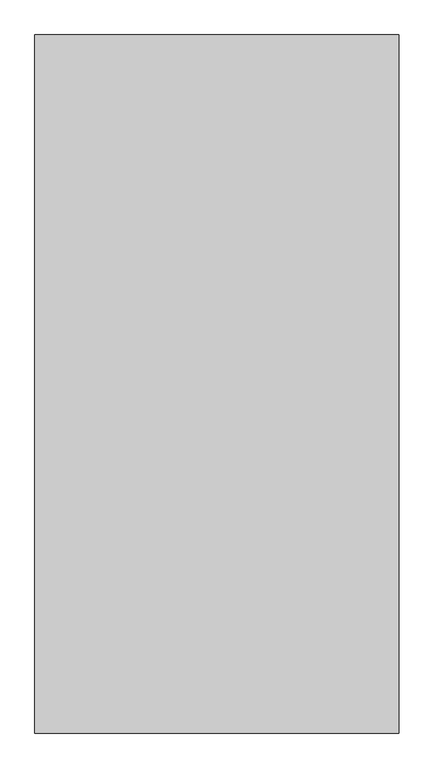
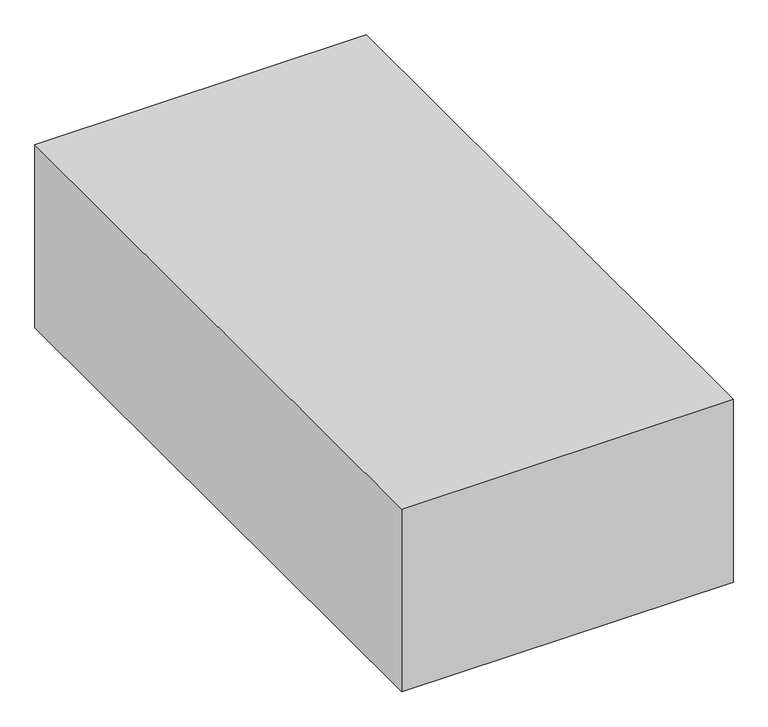
"""IFC4 building model written with IfcOpenShell, lengths in millimetres: proxy geometry, Space Planning Box_hec : Space Planning Box_hec."""

import ifcopenshell
import ifcopenshell.guid

model = None  # the IFC model being written
_history = None  # IfcOwnerHistory: only IFC2X3 demands one
_inside = {}  # id of a spatial element -> (the spatial element, [elements in it])
_under = {}  # id of a project, library or spatial element -> (it, [spatial elements below it])
_declared = {}  # id of a project -> (the project, [libraries it declares])
_typed = {}  # id of a type object -> (the type object, [elements of that type])
_made_of = {}  # id of a material, layer set ... -> (it, [elements and type objects made of it])


def new_model(schema):
    """Start an empty IFC model of exactly this schema.

    Asked for "IFC4X3", IfcOpenShell would pick the latest addendum, in which some entities
    have other attributes; the version numbers below select the first issue.
    IFC2X3 requires an IfcOwnerHistory on every rooted entity: one is made here for all.
    """
    global model, _history
    if schema == "IFC4X3":
        model = ifcopenshell.file(schema_version=(4, 3, 0, 0))
    else:
        model = ifcopenshell.file(schema=schema)
    _inside.clear()
    _under.clear()
    _declared.clear()
    _typed.clear()
    _made_of.clear()
    _history = None
    if model.schema == "IFC2X3":
        org = make("IfcOrganization", Name="unknown")
        user = make(
            "IfcPersonAndOrganization",
            ThePerson=make("IfcPerson", FamilyName="unknown"),
            TheOrganization=org,
        )
        app = make(
            "IfcApplication",
            ApplicationDeveloper=org,
            Version="unknown",
            ApplicationFullName="unknown",
            ApplicationIdentifier="unknown",
        )
        _history = make(
            "IfcOwnerHistory",
            OwningUser=user,
            OwningApplication=app,
            ChangeAction="ADDED",
            CreationDate=0,
        )
    return model


def make(cls, **values):
    """One entity of the class cls with the attributes given. An attribute that is None is left unset."""
    return model.create_entity(
        cls, **{name: value for name, value in values.items() if value is not None}
    )


def rooted(cls, **values):
    """An entity with a GlobalId (a new one), such as an element, a storey or a relation."""
    return make(cls, GlobalId=ifcopenshell.guid.new(), OwnerHistory=_history, **values)


def si_unit(unit_type, name, prefix=None):
    """IfcSIUnit, for example si_unit("LENGTHUNIT", "METRE", prefix="MILLI")."""
    return make("IfcSIUnit", UnitType=unit_type, Prefix=prefix, Name=name)


def assignment(units):
    """IfcUnitAssignment: the units of a project."""
    return None if units is None else make("IfcUnitAssignment", Units=units)


def point(xyz):
    """IfcCartesianPoint."""
    return None if xyz is None else make("IfcCartesianPoint", Coordinates=xyz)


def direction(xyz):
    """IfcDirection."""
    return None if xyz is None else make("IfcDirection", DirectionRatios=xyz)


def frame(location, z_axis=None, x_axis=None):
    """IfcAxis2Placement3D, a coordinate frame: its origin and axes. An axis left out is left unset."""
    return make(
        "IfcAxis2Placement3D",
        Location=point(location),
        Axis=direction(z_axis),
        RefDirection=direction(x_axis),
    )


def origin():
    """The frame at (0, 0, 0) with its axes left unset."""
    return frame((0.0, 0.0, 0.0))


def origin_with_axes():
    """The frame at (0, 0, 0) with the z axis (0, 0, 1) and the x axis (1, 0, 0) written out."""
    return frame((0.0, 0.0, 0.0), z_axis=(0.0, 0.0, 1.0), x_axis=(1.0, 0.0, 0.0))


def place(relative_to, where):
    """IfcLocalPlacement: puts the frame where relative to a parent placement (None: the world)."""
    return make(
        "IfcLocalPlacement", PlacementRelTo=relative_to, RelativePlacement=where
    )


def context(
    kind, dimensions, precision=None, world=None, true_north=None, identifier=None
):
    """IfcGeometricRepresentationContext, for example the 3D "Model" context."""
    return make(
        "IfcGeometricRepresentationContext",
        ContextIdentifier=identifier,
        ContextType=kind,
        CoordinateSpaceDimension=dimensions,
        Precision=precision,
        WorldCoordinateSystem=world,
        TrueNorth=true_north,
    )


def project(units=None, contexts=None):
    """IfcProject with its units and contexts."""
    return rooted(
        "IfcProject",
        Name="project",
        RepresentationContexts=contexts,
        UnitsInContext=assignment(units),
    )


def spatial(cls, under=None, at=None, **own):
    """A site, building, storey or space (cls), placed at a placement, below another one or the project."""
    s = rooted(cls, ObjectPlacement=at, **own)
    if under is not None:
        _under.setdefault(under.id(), (under, []))[1].append(s)
    return s


def polyline(points):
    """IfcPolyline through the points."""
    return make("IfcPolyline", Points=[point(p) for p in points])


def outline(outer, holes=None, kind="AREA"):
    """IfcArbitraryClosedProfileDef: a profile drawn as a closed curve; with holes, ...WithVoids."""
    if holes is None:
        return make("IfcArbitraryClosedProfileDef", ProfileType=kind, OuterCurve=outer)
    return make(
        "IfcArbitraryProfileDefWithVoids",
        ProfileType=kind,
        OuterCurve=outer,
        InnerCurves=holes,
    )


def extrude(swept, where, along, depth):
    """IfcExtrudedAreaSolid: the profile swept, set in the frame where, extruded along a direction by depth."""
    return make(
        "IfcExtrudedAreaSolid",
        SweptArea=swept,
        Position=where,
        ExtrudedDirection=direction(along),
        Depth=depth,
    )


def shape(context_of_items, identifier, shape_type, items):
    """IfcShapeRepresentation: the items that make up one representation, for example the "Body"."""
    return make(
        "IfcShapeRepresentation",
        ContextOfItems=context_of_items,
        RepresentationIdentifier=identifier,
        RepresentationType=shape_type,
        Items=items,
    )


def source(mapping_origin, context_of_items, identifier, shape_type, items):
    """IfcRepresentationMap: a shape defined once, which mapped items show again and again."""
    return make(
        "IfcRepresentationMap",
        MappingOrigin=mapping_origin,
        MappedRepresentation=shape(context_of_items, identifier, shape_type, items),
    )


def transform(
    local_origin,
    x_axis=None,
    y_axis=None,
    z_axis=None,
    scale=None,
    scale2=None,
    scale3=None,
    uniform=True,
):
    """IfcCartesianTransformationOperator3D, or its non-uniform kind. x_axis, y_axis, z_axis: its Axis1, 2, 3."""
    if uniform:
        return make(
            "IfcCartesianTransformationOperator3D",
            Axis1=direction(x_axis),
            Axis2=direction(y_axis),
            LocalOrigin=point(local_origin),
            Scale=scale,
            Axis3=direction(z_axis),
        )
    return make(
        "IfcCartesianTransformationOperator3DnonUniform",
        Axis1=direction(x_axis),
        Axis2=direction(y_axis),
        LocalOrigin=point(local_origin),
        Scale=scale,
        Axis3=direction(z_axis),
        Scale2=scale2,
        Scale3=scale3,
    )


def mapped(mapping_source, mapping_target):
    """IfcMappedItem: shows the shape of a source again, moved by a transform."""
    return make(
        "IfcMappedItem", MappingSource=mapping_source, MappingTarget=mapping_target
    )


def made_of(thing, what):
    """Note that an element or type object is made of a material, layer set ...; save() writes the relation."""
    if what is not None:
        _made_of.setdefault(what.id(), (what, []))[1].append(thing)
    return thing


def element(
    cls,
    number,
    at=None,
    inside=None,
    cuts=None,
    type_object=None,
    material=None,
    context=None,
    identifier="Body",
    shape_type=None,
    held_by="IfcProductDefinitionShape",
    body=None,
    shapes=None,
    **own,
):
    """One element of the class cls, such as IfcWall. Its Tag is "e" and its number.

    at: its placement. inside: the storey or other place that contains it. cuts: it is an
    opening in that element (IfcRelVoidsElement). A single representation is given by context,
    identifier, shape_type and body (its items); several are given by shapes. held_by: the class
    of the entity that holds the representations. save() writes the other relations.
    """
    e = rooted(cls, Tag="e%d" % number, ObjectPlacement=at, **own)
    if body is not None:
        shapes = [shape(context, identifier, shape_type, body)]
    if shapes is not None:
        e.Representation = make(held_by, Representations=shapes)
    if inside is not None:
        _inside.setdefault(inside.id(), (inside, []))[1].append(e)
    if cuts is not None:
        rooted(
            "IfcRelVoidsElement", RelatingBuildingElement=cuts, RelatedOpeningElement=e
        )
    if type_object is not None:
        _typed.setdefault(type_object.id(), (type_object, []))[1].append(e)
    return made_of(e, material)


def aggregate(whole, parts):
    """IfcRelAggregates: a whole, such as a stair, and the parts it consists of."""
    return rooted("IfcRelAggregates", RelatingObject=whole, RelatedObjects=parts)


def save(model, path):
    """Write the relations noted so far, then the file.

    IfcRelAggregates (storeys below a building ...), IfcRelContainedInSpatialStructure (elements
    in a storey), IfcRelDefinesByType, IfcRelAssociatesMaterial and IfcRelDeclares: one each for
    every whole, place, type object, material and project.
    """
    for whole, parts in _under.values():
        aggregate(whole, parts)
    for where, things in _inside.values():
        rooted(
            "IfcRelContainedInSpatialStructure",
            RelatedElements=things,
            RelatingStructure=where,
        )
    for kind, things in _typed.values():
        rooted("IfcRelDefinesByType", RelatedObjects=things, RelatingType=kind)
    for what, things in _made_of.values():
        rooted("IfcRelAssociatesMaterial", RelatedObjects=things, RelatingMaterial=what)
    for by, libraries in _declared.values():
        rooted("IfcRelDeclares", RelatingContext=by, RelatedDefinitions=libraries)
    model.write(path)


def generic_models_ccc8c8c2(model_context):
    return source(origin(), model_context, "Body", "SweptSolid", [
        extrude(outline(polyline([(3000.0, 5750.0), (3000.0, -5750.0), (-3000.0, -5750.0), (-3000.0, 5750.0), (3000.0, 5750.0)])), origin_with_axes(), (0.0, 0.0, 1.0), 3500.0),
    ])


if __name__ == "__main__":
    model = new_model("IFC4")
    model_context = context("Model", 3, world=origin())
    ifc_project = project(units=[si_unit("LENGTHUNIT", "METRE", prefix="MILLI")], contexts=[model_context])
    site = spatial("IfcSite", under=ifc_project)
    building = spatial("IfcBuilding", under=site)
    placement = place(None, origin())
    generic_models_shape = generic_models_ccc8c8c2(model_context)
    element("IfcBuildingElementProxy", 1, Name="Space Planning Box_hec : Space Planning Box_hec", ObjectType="Space Planning Box_hec : Space Planning Box_hec", at=placement, inside=building, context=model_context, shape_type="MappedRepresentation", body=[
        mapped(generic_models_shape, transform((0.0, 0.0, 0.0), x_axis=(1.0, 0.0, 0.0), y_axis=(0.0, 1.0, 0.0), z_axis=(0.0, 0.0, 1.0))),
    ])
    save(model, "model.ifc")

# Revit data of these elements
# Type "Space Planning Box_hec : Space Planning Box_hec"
#   Type Comments = "..."
#   Room Name [instance default] = "?"
#   Interior Finish [instance default] = ""
#   Exterior Finish [instance default] = ""
#   Department [instance default] = ""
#   Assembly Code = "..."
#   ceiling height [instance default] = 0
#   Width [instance default] = 1524 mm
#   Program Area [instance default] = 0.00 m²
#   Length [instance default] = 1524 mm
#   Height [instance default] = 1524 mm
#   Area [instance default] = 2.32258 m²
#   Fill Color [instance default] = Cyan
#   Default Elevation = 0
# Element 1 (IfcBuildingElementProxy, "Space Planning Box_hec : Space Planning Box_hec")
#   Room Name = "Meeting Room-1"
#   Exterior Finish = "RF1..N/A,,EW1..EW2..N/A"
#   Department = "AR"
#   Width = 6000 mm
#   Program Area = 69.00 m²
#   Length = 11500 mm
#   Height = 3500 mm
#   Area = 69.00 m²
#   Materials on its faces: "Cyan"
# Materials
#   "Cyan": class "Generic", colour RGB 0 255 255, transparency 0.2, Cost = 0
